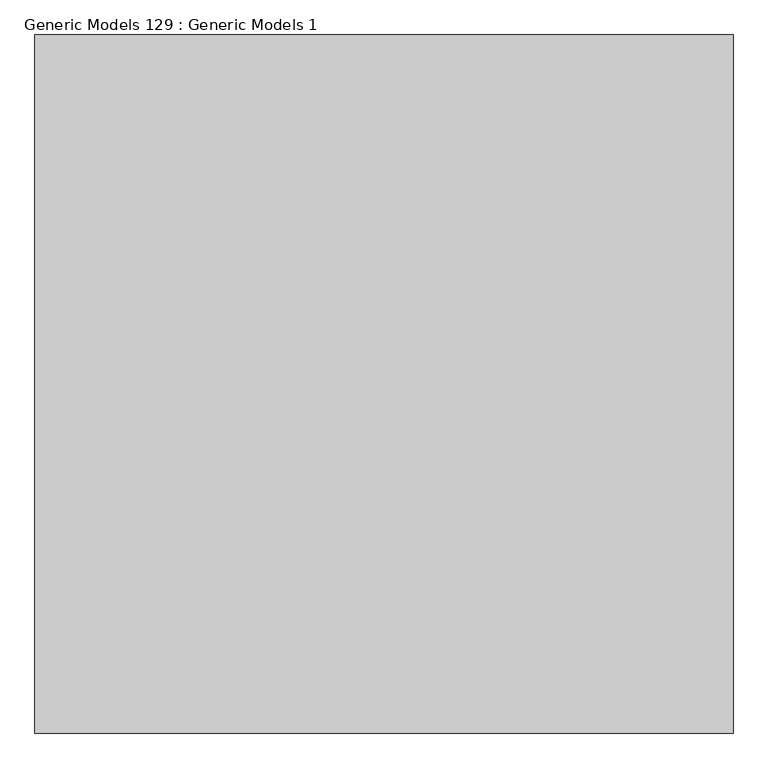
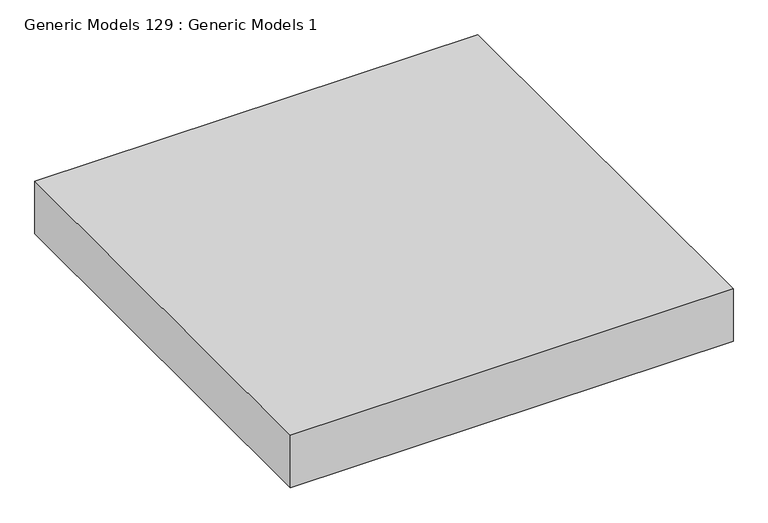
"""IFC4 building model written with IfcOpenShell, lengths in millimetres: proxy geometry, Generic Models 129 : Generic Models 1."""

import ifcopenshell
import ifcopenshell.guid

model = None  # the IFC model being written
_history = None  # IfcOwnerHistory: only IFC2X3 demands one
_inside = {}  # id of a spatial element -> (the spatial element, [elements in it])
_under = {}  # id of a project, library or spatial element -> (it, [spatial elements below it])
_declared = {}  # id of a project -> (the project, [libraries it declares])
_typed = {}  # id of a type object -> (the type object, [elements of that type])
_made_of = {}  # id of a material, layer set ... -> (it, [elements and type objects made of it])


def new_model(schema):
    """Start an empty IFC model of exactly this schema.

    Asked for "IFC4X3", IfcOpenShell would pick the latest addendum, in which some entities
    have other attributes; the version numbers below select the first issue.
    IFC2X3 requires an IfcOwnerHistory on every rooted entity: one is made here for all.
    """
    global model, _history
    if schema == "IFC4X3":
        model = ifcopenshell.file(schema_version=(4, 3, 0, 0))
    else:
        model = ifcopenshell.file(schema=schema)
    _inside.clear()
    _under.clear()
    _declared.clear()
    _typed.clear()
    _made_of.clear()
    _history = None
    if model.schema == "IFC2X3":
        org = make("IfcOrganization", Name="unknown")
        user = make(
            "IfcPersonAndOrganization",
            ThePerson=make("IfcPerson", FamilyName="unknown"),
            TheOrganization=org,
        )
        app = make(
            "IfcApplication",
            ApplicationDeveloper=org,
            Version="unknown",
            ApplicationFullName="unknown",
            ApplicationIdentifier="unknown",
        )
        _history = make(
            "IfcOwnerHistory",
            OwningUser=user,
            OwningApplication=app,
            ChangeAction="ADDED",
            CreationDate=0,
        )
    return model


def make(cls, **values):
    """One entity of the class cls with the attributes given. An attribute that is None is left unset."""
    return model.create_entity(
        cls, **{name: value for name, value in values.items() if value is not None}
    )


def rooted(cls, **values):
    """An entity with a GlobalId (a new one), such as an element, a storey or a relation."""
    return make(cls, GlobalId=ifcopenshell.guid.new(), OwnerHistory=_history, **values)


def si_unit(unit_type, name, prefix=None):
    """IfcSIUnit, for example si_unit("LENGTHUNIT", "METRE", prefix="MILLI")."""
    return make("IfcSIUnit", UnitType=unit_type, Prefix=prefix, Name=name)


def assignment(units):
    """IfcUnitAssignment: the units of a project."""
    return None if units is None else make("IfcUnitAssignment", Units=units)


def point(xyz):
    """IfcCartesianPoint."""
    return None if xyz is None else make("IfcCartesianPoint", Coordinates=xyz)


def direction(xyz):
    """IfcDirection."""
    return None if xyz is None else make("IfcDirection", DirectionRatios=xyz)


def frame(location, z_axis=None, x_axis=None):
    """IfcAxis2Placement3D, a coordinate frame: its origin and axes. An axis left out is left unset."""
    return make(
        "IfcAxis2Placement3D",
        Location=point(location),
        Axis=direction(z_axis),
        RefDirection=direction(x_axis),
    )


def origin():
    """The frame at (0, 0, 0) with its axes left unset."""
    return frame((0.0, 0.0, 0.0))


def place(relative_to, where):
    """IfcLocalPlacement: puts the frame where relative to a parent placement (None: the world)."""
    return make(
        "IfcLocalPlacement", PlacementRelTo=relative_to, RelativePlacement=where
    )


def context(
    kind, dimensions, precision=None, world=None, true_north=None, identifier=None
):
    """IfcGeometricRepresentationContext, for example the 3D "Model" context."""
    return make(
        "IfcGeometricRepresentationContext",
        ContextIdentifier=identifier,
        ContextType=kind,
        CoordinateSpaceDimension=dimensions,
        Precision=precision,
        WorldCoordinateSystem=world,
        TrueNorth=true_north,
    )


def project(units=None, contexts=None):
    """IfcProject with its units and contexts."""
    return rooted(
        "IfcProject",
        Name="project",
        RepresentationContexts=contexts,
        UnitsInContext=assignment(units),
    )


def spatial(cls, under=None, at=None, **own):
    """A site, building, storey or space (cls), placed at a placement, below another one or the project."""
    s = rooted(cls, ObjectPlacement=at, **own)
    if under is not None:
        _under.setdefault(under.id(), (under, []))[1].append(s)
    return s


def polyline(points):
    """IfcPolyline through the points."""
    return make("IfcPolyline", Points=[point(p) for p in points])


def outline(outer, holes=None, kind="AREA"):
    """IfcArbitraryClosedProfileDef: a profile drawn as a closed curve; with holes, ...WithVoids."""
    if holes is None:
        return make("IfcArbitraryClosedProfileDef", ProfileType=kind, OuterCurve=outer)
    return make(
        "IfcArbitraryProfileDefWithVoids",
        ProfileType=kind,
        OuterCurve=outer,
        InnerCurves=holes,
    )


def extrude(swept, where, along, depth):
    """IfcExtrudedAreaSolid: the profile swept, set in the frame where, extruded along a direction by depth."""
    return make(
        "IfcExtrudedAreaSolid",
        SweptArea=swept,
        Position=where,
        ExtrudedDirection=direction(along),
        Depth=depth,
    )


def shape(context_of_items, identifier, shape_type, items):
    """IfcShapeRepresentation: the items that make up one representation, for example the "Body"."""
    return make(
        "IfcShapeRepresentation",
        ContextOfItems=context_of_items,
        RepresentationIdentifier=identifier,
        RepresentationType=shape_type,
        Items=items,
    )


def source(mapping_origin, context_of_items, identifier, shape_type, items):
    """IfcRepresentationMap: a shape defined once, which mapped items show again and again."""
    return make(
        "IfcRepresentationMap",
        MappingOrigin=mapping_origin,
        MappedRepresentation=shape(context_of_items, identifier, shape_type, items),
    )


def transform(
    local_origin,
    x_axis=None,
    y_axis=None,
    z_axis=None,
    scale=None,
    scale2=None,
    scale3=None,
    uniform=True,
):
    """IfcCartesianTransformationOperator3D, or its non-uniform kind. x_axis, y_axis, z_axis: its Axis1, 2, 3."""
    if uniform:
        return make(
            "IfcCartesianTransformationOperator3D",
            Axis1=direction(x_axis),
            Axis2=direction(y_axis),
            LocalOrigin=point(local_origin),
            Scale=scale,
            Axis3=direction(z_axis),
        )
    return make(
        "IfcCartesianTransformationOperator3DnonUniform",
        Axis1=direction(x_axis),
        Axis2=direction(y_axis),
        LocalOrigin=point(local_origin),
        Scale=scale,
        Axis3=direction(z_axis),
        Scale2=scale2,
        Scale3=scale3,
    )


def mapped(mapping_source, mapping_target):
    """IfcMappedItem: shows the shape of a source again, moved by a transform."""
    return make(
        "IfcMappedItem", MappingSource=mapping_source, MappingTarget=mapping_target
    )


def made_of(thing, what):
    """Note that an element or type object is made of a material, layer set ...; save() writes the relation."""
    if what is not None:
        _made_of.setdefault(what.id(), (what, []))[1].append(thing)
    return thing


def element(
    cls,
    number,
    at=None,
    inside=None,
    cuts=None,
    type_object=None,
    material=None,
    context=None,
    identifier="Body",
    shape_type=None,
    held_by="IfcProductDefinitionShape",
    body=None,
    shapes=None,
    **own,
):
    """One element of the class cls, such as IfcWall. Its Tag is "e" and its number.

    at: its placement. inside: the storey or other place that contains it. cuts: it is an
    opening in that element (IfcRelVoidsElement). A single representation is given by context,
    identifier, shape_type and body (its items); several are given by shapes. held_by: the class
    of the entity that holds the representations. save() writes the other relations.
    """
    e = rooted(cls, Tag="e%d" % number, ObjectPlacement=at, **own)
    if body is not None:
        shapes = [shape(context, identifier, shape_type, body)]
    if shapes is not None:
        e.Representation = make(held_by, Representations=shapes)
    if inside is not None:
        _inside.setdefault(inside.id(), (inside, []))[1].append(e)
    if cuts is not None:
        rooted(
            "IfcRelVoidsElement", RelatingBuildingElement=cuts, RelatedOpeningElement=e
        )
    if type_object is not None:
        _typed.setdefault(type_object.id(), (type_object, []))[1].append(e)
    return made_of(e, material)


def aggregate(whole, parts):
    """IfcRelAggregates: a whole, such as a stair, and the parts it consists of."""
    return rooted("IfcRelAggregates", RelatingObject=whole, RelatedObjects=parts)


def save(model, path):
    """Write the relations noted so far, then the file.

    IfcRelAggregates (storeys below a building ...), IfcRelContainedInSpatialStructure (elements
    in a storey), IfcRelDefinesByType, IfcRelAssociatesMaterial and IfcRelDeclares: one each for
    every whole, place, type object, material and project.
    """
    for whole, parts in _under.values():
        aggregate(whole, parts)
    for where, things in _inside.values():
        rooted(
            "IfcRelContainedInSpatialStructure",
            RelatedElements=things,
            RelatingStructure=where,
        )
    for kind, things in _typed.values():
        rooted("IfcRelDefinesByType", RelatedObjects=things, RelatingType=kind)
    for what, things in _made_of.values():
        rooted("IfcRelAssociatesMaterial", RelatedObjects=things, RelatingMaterial=what)
    for by, libraries in _declared.values():
        rooted("IfcRelDeclares", RelatingContext=by, RelatedDefinitions=libraries)
    model.write(path)


def generic_models_129_generic_models_1_8999e842(model_context):
    return source(origin(), model_context, "Body", "SweptSolid", [
        extrude(outline(polyline([(47499.4360531, 0.0), (46280.2360531, 0.0), (46280.2360531, 1219.2), (47499.4360531, 1219.2), (47499.4360531, 0.0)])), frame((0.0, 0.0, -378.376067), z_axis=(0.0, 0.0, 1.0), x_axis=(1.0, 0.0, 0.0)), (0.0, 0.0, 1.0), 152.4),
    ])


if __name__ == "__main__":
    model = new_model("IFC4")
    model_context = context("Model", 3, world=origin())
    ifc_project = project(units=[si_unit("LENGTHUNIT", "METRE", prefix="MILLI")], contexts=[model_context])
    site = spatial("IfcSite", under=ifc_project)
    building = spatial("IfcBuilding", under=site)
    placement = place(None, origin())
    generic_models_129_generic_models_1_shape = generic_models_129_generic_models_1_8999e842(model_context)
    element("IfcBuildingElementProxy", 1, Name="Generic Models 129 : Generic Models 1", ObjectType="Generic Models 129 : Generic Models 1", at=placement, inside=building, context=model_context, shape_type="MappedRepresentation", body=[
        mapped(generic_models_129_generic_models_1_shape, transform((0.0, 0.0, 0.0), x_axis=(1.0, 0.0, 0.0), y_axis=(0.0, 1.0, 0.0), z_axis=(0.0, 0.0, 1.0))),
    ])
    save(model, "model.ifc")

# Revit data of these elements
# Element 1 (IfcBuildingElementProxy, "Generic Models 129 : Generic Models 1")
#   Materials on its faces: "EXISTING SLAB"
# Materials
#   "EXISTING SLAB": class "Concrete", colour RGB 129 132 118, transparency 0, Description = "Lightweight concrete", Cost = 0
